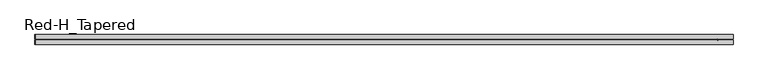
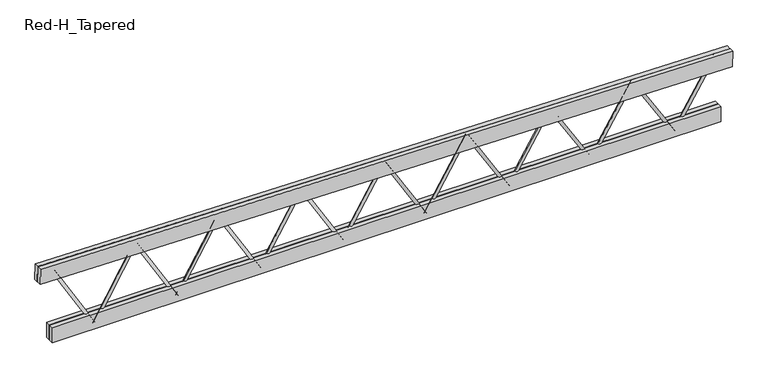
"""IFC4 building model written with IfcOpenShell, lengths in millimetres: beam geometry, Construction_Frames_RedBuilt_Openweb_Red-H_Tapered : Red-H_Tapered."""

from ifc_helpers import new_model, si_unit, point, frame, origin, origin_2d, place, context, project, spatial, polyline, circle_curve, trimmed, segment, composite_curve, outline, extrude, source, transform, mapped, element, save


def red_h_tapered_639e8230(model_context):
    return source(origin(), model_context, "Body", "SweptSolid", [
        extrude(outline(composite_curve([segment(trimmed(circle_curve(origin_2d(), 12.7), [point((0.0, 12.7))], [point((0.0, -12.7))], False, "CARTESIAN"), True, "CONTINUOUS"), segment(trimmed(circle_curve(origin_2d(), 12.7), [point((0.0, -12.7))], [point((0.0, 12.7))], False, "CARTESIAN"), True, "CONTINUOUS")], self_intersect=False)), frame((2514.6356775, 0.0, -367.0101562), z_axis=(0.5238075847033234, 0.0, 0.8518366123895301), x_axis=(0.0, -1.0, 0.0)), (0.0, 0.0, 1.0), 685.812269),
        extrude(outline(composite_curve([segment(trimmed(circle_curve(origin_2d(), 12.7), [point((0.0, -12.7))], [point((0.0, 12.6999999))], False, "CARTESIAN"), True, "CONTINUOUS"), segment(trimmed(circle_curve(origin_2d(), 12.7), [point((0.0, 12.6999999))], [point((0.0, -12.7))], False, "CARTESIAN"), True, "CONTINUOUS")], self_intersect=False)), frame((2514.6356775, 0.0, -367.0101562), z_axis=(-0.5212365661564216, 0.0, 0.8534122345627947), x_axis=(0.0, -1.0, 0.0)), (0.0, 0.0, 1.0), 689.1950633),
        extrude(outline(composite_curve([segment(trimmed(circle_curve(origin_2d(), 12.7), [point((0.0, 12.7))], [point((0.0, -12.6999999))], False, "CARTESIAN"), True, "CONTINUOUS"), segment(trimmed(circle_curve(origin_2d(), 12.7), [point((0.0, -12.6999999))], [point((0.0, 12.7))], False, "CARTESIAN"), True, "CONTINUOUS")], self_intersect=False)), frame((1796.168341, 0.0, -367.0101562), z_axis=(0.5212365661564208, 0.0, 0.8534122345627951), x_axis=(0.0, -1.0, 0.0)), (0.0, 0.0, 1.0), 689.1950633),
        extrude(outline(composite_curve([segment(trimmed(circle_curve(origin_2d(), 12.7), [point((0.0, -12.7))], [point((0.0, 12.7000001))], False, "CARTESIAN"), True, "CONTINUOUS"), segment(trimmed(circle_curve(origin_2d(), 12.7), [point((0.0, 12.7000001))], [point((0.0, -12.7))], False, "CARTESIAN"), True, "CONTINUOUS")], self_intersect=False)), frame((1796.168341, 0.0, -367.0101562), z_axis=(-0.5186860157662654, 0.0, 0.854964804567134), x_axis=(0.0, -1.0, 0.0)), (0.0, 0.0, 1.0), 692.584063),
        extrude(outline(composite_curve([segment(trimmed(circle_curve(origin_2d(), 12.7), [point((0.0, 12.7))], [point((0.0, -12.7))], False, "CARTESIAN"), True, "CONTINUOUS"), segment(trimmed(circle_curve(origin_2d(), 12.7), [point((0.0, -12.7))], [point((0.0, 12.7))], False, "CARTESIAN"), True, "CONTINUOUS")], self_intersect=False)), frame((1077.7010046, 0.0, -367.0101562), z_axis=(0.5186860157662644, 0.0, 0.8549648045671345), x_axis=(0.0, -1.0, 0.0)), (0.0, 0.0, 1.0), 692.584063),
        extrude(outline(composite_curve([segment(trimmed(circle_curve(origin_2d(), 12.7), [point((0.0, -12.7))], [point((0.0, 12.7))], False, "CARTESIAN"), True, "CONTINUOUS"), segment(trimmed(circle_curve(origin_2d(), 12.7), [point((0.0, 12.7))], [point((0.0, -12.7))], False, "CARTESIAN"), True, "CONTINUOUS")], self_intersect=False)), frame((1077.7010046, 0.0, -367.0101562), z_axis=(-0.5161557699811348, 0.0, 0.8564947291812028), x_axis=(0.0, -1.0, 0.0)), (0.0, 0.0, 1.0), 695.9791774),
        extrude(outline(composite_curve([segment(trimmed(circle_curve(origin_2d(), 12.7), [point((0.0, 12.7))], [point((0.0, -12.7))], False, "CARTESIAN"), True, "CONTINUOUS"), segment(trimmed(circle_curve(origin_2d(), 12.7), [point((0.0, -12.7))], [point((0.0, 12.7))], False, "CARTESIAN"), True, "CONTINUOUS")], self_intersect=False)), frame((359.2336682, 0.0, -367.0101562), z_axis=(0.5161557699811353, 0.0, 0.8564947291812025), x_axis=(0.0, -1.0, 0.0)), (0.0, 0.0, 1.0), 695.9791774),
        extrude(outline(composite_curve([segment(trimmed(circle_curve(origin_2d(), 12.7), [point((0.0, -12.7000001))], [point((0.0, 12.7))], False, "CARTESIAN"), True, "CONTINUOUS"), segment(trimmed(circle_curve(origin_2d(), 12.7), [point((0.0, 12.7))], [point((0.0, -12.7000001))], False, "CARTESIAN"), True, "CONTINUOUS")], self_intersect=False)), frame((359.2336682, 0.0, -367.0101562), z_axis=(-0.5136456648662082, 0.0, 0.8580024073183892), x_axis=(0.0, -1.0, 0.0)), (0.0, 0.0, 1.0), 699.3803176),
        extrude(outline(composite_curve([segment(trimmed(circle_curve(origin_2d(), 12.7), [point((0.0, -12.7))], [point((0.0, 12.7000001))], False, "CARTESIAN"), True, "CONTINUOUS"), segment(trimmed(circle_curve(origin_2d(), 12.7), [point((0.0, 12.7000001))], [point((0.0, -12.7))], False, "CARTESIAN"), True, "CONTINUOUS")], self_intersect=False)), frame((-359.2336682, 0.0, -367.0101562), z_axis=(0.5136456648661768, 0.0, 0.858002407318408), x_axis=(0.0, -1.0, 0.0)), (0.0, 0.0, 1.0), 699.3803176),
        extrude(outline(composite_curve([segment(trimmed(circle_curve(origin_2d(), 12.7), [point((0.0, 12.7))], [point((0.0, -12.7))], False, "CARTESIAN"), True, "CONTINUOUS"), segment(trimmed(circle_curve(origin_2d(), 12.7), [point((0.0, -12.7))], [point((0.0, 12.7))], False, "CARTESIAN"), True, "CONTINUOUS")], self_intersect=False)), frame((-359.2336682, 0.0, -367.0101562), z_axis=(-0.5111555362037679, 0.0, 0.8594882301743513), x_axis=(0.0, -1.0, 0.0)), (0.0, 0.0, 1.0), 702.7873959),
        extrude(outline(composite_curve([segment(trimmed(circle_curve(origin_2d(), 12.7), [point((0.0, -12.7000001))], [point((0.0, 12.7))], False, "CARTESIAN"), True, "CONTINUOUS"), segment(trimmed(circle_curve(origin_2d(), 12.7), [point((0.0, 12.7))], [point((0.0, -12.7000001))], False, "CARTESIAN"), True, "CONTINUOUS")], self_intersect=False)), frame((-1077.7010046, 0.0, -367.0101562), z_axis=(0.5111555362037662, 0.0, 0.8594882301743523), x_axis=(0.0, -1.0, 0.0)), (0.0, 0.0, 1.0), 702.7873959),
        extrude(outline(composite_curve([segment(trimmed(circle_curve(origin_2d(), 12.7), [point((0.0, 12.7))], [point((0.0, -12.7))], False, "CARTESIAN"), True, "CONTINUOUS"), segment(trimmed(circle_curve(origin_2d(), 12.7), [point((0.0, -12.7))], [point((0.0, 12.7))], False, "CARTESIAN"), True, "CONTINUOUS")], self_intersect=False)), frame((-1077.7010046, 0.0, -367.0101562), z_axis=(-0.5086852195886402, 0.0, 0.8609525813725497), x_axis=(0.0, -1.0, 0.0)), (0.0, 0.0, 1.0), 706.2003266),
        extrude(outline(composite_curve([segment(trimmed(circle_curve(origin_2d(), 12.7), [point((0.0, -12.7))], [point((0.0, 12.6999999))], False, "CARTESIAN"), True, "CONTINUOUS"), segment(trimmed(circle_curve(origin_2d(), 12.7), [point((0.0, 12.6999999))], [point((0.0, -12.7))], False, "CARTESIAN"), True, "CONTINUOUS")], self_intersect=False)), frame((-1796.168341, 0.0, -367.0101562), z_axis=(0.5086852195886533, 0.0, 0.860952581372542), x_axis=(0.0, -1.0, 0.0)), (0.0, 0.0, 1.0), 706.2003266),
        extrude(outline(composite_curve([segment(trimmed(circle_curve(origin_2d(), 12.7), [point((0.0, 12.6999999))], [point((0.0, -12.7000001))], False, "CARTESIAN"), True, "CONTINUOUS"), segment(trimmed(circle_curve(origin_2d(), 12.7), [point((0.0, -12.7000001))], [point((0.0, 12.6999999))], False, "CARTESIAN"), True, "CONTINUOUS")], self_intersect=False)), frame((-1796.168341, 0.0, -367.0101562), z_axis=(-0.5062345505185007, 0.0, 0.8623958371080716), x_axis=(0.0, -1.0, 0.0)), (0.0, 0.0, 1.0), 709.6190251),
        extrude(outline(composite_curve([segment(trimmed(circle_curve(origin_2d(), 12.7), [point((0.0, -12.6999999))], [point((0.0, 12.7000001))], False, "CARTESIAN"), True, "CONTINUOUS"), segment(trimmed(circle_curve(origin_2d(), 12.7), [point((0.0, 12.7000001))], [point((0.0, -12.6999999))], False, "CARTESIAN"), True, "CONTINUOUS")], self_intersect=False)), frame((-2514.6356775, 0.0, -367.0101562), z_axis=(0.506234550518489, 0.0, 0.8623958371080784), x_axis=(0.0, -1.0, 0.0)), (0.0, 0.0, 1.0), 709.6190251),
        extrude(outline(composite_curve([segment(trimmed(circle_curve(origin_2d(), 12.7), [point((0.0, 12.7))], [point((0.0, -12.7))], False, "CARTESIAN"), True, "CONTINUOUS"), segment(trimmed(circle_curve(origin_2d(), 12.7), [point((0.0, -12.7))], [point((0.0, 12.7))], False, "CARTESIAN"), True, "CONTINUOUS")], self_intersect=False)), frame((-2514.6356775, 0.0, -367.0101562), z_axis=(-0.5038033644797567, 0.0, 0.8638183662893939), x_axis=(0.0, -1.0, 0.0)), (0.0, 0.0, 1.0), 713.0434085),
        extrude(outline(polyline([(-2899.2693457, -41.275), (-2899.2693457, -3.175), (2899.2693457, -3.175), (2899.2693457, -41.275), (-2899.2693457, -41.275)])), frame((0.0, 0.0, -386.0601562), z_axis=(0.0, 0.0, 1.0), x_axis=(1.0, 0.0, 0.0)), (0.0, 0.0, 1.0), 139.7),
        extrude(outline(polyline([(-2899.2693457, 3.175), (-2899.2693457, 41.275), (2899.2693457, 41.275), (2899.2693457, 3.175), (-2899.2693457, 3.175)])), frame((0.0, 0.0, -386.0601562), z_axis=(0.0, 0.0, 1.0), x_axis=(1.0, 0.0, 0.0)), (0.0, 0.0, 1.0), 139.7),
        extrude(outline(polyline([(0.0, -38.1), (0.0, 0.0), (6002.5985939, 0.0), (6002.5985939, -38.1), (0.0, -38.1)])), frame((-3003.2339083, -3.175, 185.4598565), z_axis=(0.016926002698829056, 0.0, 0.9998567449553157), x_axis=(0.9998567449553157, 0.0, -0.016926002698829056)), (0.0, 0.0, 1.0), 139.7),
        extrude(outline(polyline([(0.0, -38.1), (0.0, 0.0), (6002.5985939, 0.0), (6002.5985939, -38.1), (0.0, -38.1)])), frame((-3003.2339083, 41.275, 185.4598565), z_axis=(0.016926002698829056, 0.0, 0.9998567449553157), x_axis=(0.9998567449553157, 0.0, -0.016926002698829056)), (0.0, 0.0, 1.0), 139.7),
    ])


if __name__ == "__main__":
    model = new_model("IFC4")
    model_context = context("Model", 3, world=origin())
    ifc_project = project(units=[si_unit("LENGTHUNIT", "METRE", prefix="MILLI")], contexts=[model_context])
    site = spatial("IfcSite", under=ifc_project)
    building = spatial("IfcBuilding", under=site)
    placement = place(None, origin())
    red_h_tapered_shape = red_h_tapered_639e8230(model_context)
    element("IfcBeam", 1, ObjectType="Construction_Frames_RedBuilt_Openweb_Red-H_Tapered : Red-H_Tapered", at=placement, inside=building, context=model_context, shape_type="MappedRepresentation", body=[
        mapped(red_h_tapered_shape, transform((0.0, 0.0, 0.0), x_axis=(1.0, 0.0, 0.0), y_axis=(0.0, 1.0, 0.0), z_axis=(0.0, 0.0, 1.0))),
    ])
    save(model, "model.ifc")

# Revit data of these elements
# Type "Construction_Frames_RedBuilt_Openweb_Red-H_Tapered : Red-H_Tapered"
#   Youtube clip = ""
#   Weight Net (Kg) = "0"
#   Webs = "Up to 2\" diameter tubular steel"
#   Uniformat II Description = ""
#   Uniformat II Code = ""
#   Uniclass 2015 Name = "Softwood trusses"
#   Uniclass 2015 Code = "Pr_20_85_90_81"
#   Uniclass 2.0 Description = "Structural Framing Systems"
#   Uniclass 2.0 Code = "SS-15-10-75"
#   Uniclass 1.4 Description = "Trusses"
#   Uniclass 1.4 Code = "L3523"
#   UNSPSC Code = "30103606"
#   Technical description = "http://www.redbuilt.com/reference/literature-and-other-resources"
#   Region South America = "None"
#   Region Oceania = "None"
#   Region North America = "US"
#   Region Middle East = "None"
#   Region Europe = "None"
#   Region Asia = "None"
#   Region Antarctica = "None"
#   Region Africa = "None"
#   QR code = "http://bimobject.com/redbuilt/product/redbuilt-0003"
#   Product url = "http://www.redbuilt.com/products/default.aspx?id=2"
#   Product group = "Wood Trusses"
#   Product family = "Construction"
#   Product data url = "https://bimobject.com/redbuilt/product/redbuilt-0003"
#   Product certification = ""
#   Product SKU = "redbuilt-0003"
#   Product Page URL = "http://www.redbuilt.com/commercial-systems/red-m-red-h-open-web-trusses"
#   Product Guid = "2c5793f2-6ffb-4665-b825-cf90c048e711"
#   Product Documentation Link = "http://www.redbuilt.com/documents/OW_Guide_2017_07_LowRes_wLinks.pdf"
#   OmniClass Description = "Wood Trusses"
#   OmniClass Code = "23-13 35 19 13 17"
#   NBS Reference Description = ""
#   NBS Reference Code = ""
#   Material secondary = "Steel"
#   Material main = "CHARRED WOOD"
#   Masterformat 2014 Description = "Metal-Web Wood Joists"
#   Masterformat 2014 Code = "06 17 36"
#   Manufacturer name = "RedBuilt"
#   Manufacturer country = "United States"
#   Installation instructions = "http://www.redbuilt.com/documents/Installation_Sheets_Open-Web.pdf"
#   IFC Classification = ""
#   EAN code = ""
#   Design country = "United States"
#   Product Information = "http://redbuilt.com/products/default.aspx?id=2"
#   Model = "Red-H-Tapered"
#   Manufacturer URL = "http://redbuilt.com/"
#   Manufacturer = "RedBuilt™"
#   Description = "Open Web Truss"
#   Date of publishing = "8/17/2010"
#   Contact us = "http://redbuilt.com/contact/"
#   Chords = "Double 1½\" x 5½\" MSR lumber"
#   COBIe Type Category = ""
#   Brand url = "http://www.redbuilt.com"
#   BIMobject main category code = "construction"
#   BIMobject main category = "Construction"
#   BIMobject category code = "construction-frames-trusses"
#   BIMobject category = "Frames & Trusses"
#   Web Radius = 0' - 0 1/2"
#   Web Layout Offset Start [instance default] = 0' - 5"
#   Web Layout Offset End [instance default] = 0' - 5"
#   Web Diameter = 0' - 1"
#   TotalLength [instance default] = 20' - 0"
#   Span Minimum = 4' - 0"
#   Span Maximum = 70' - 0"
#   Span Limit [instance default] = 20' - 0"
#   Nominal width = 0' - 0"
#   Nominal height = 0' - 0"
#   Inner Depth Top [instance default] = 0' - 2.76372"
#   Depth Start [instance default] = 6' - 0"
#   Top Chord Length [instance default] = 20' - 1.19701"
#   TC Extension Start Aux [instance default] = 0' - 0"
#   TC Extension End Aux [instance default] = 0' - 0"
#   T-B Chord Length Difference L [instance default] = 0' - 4"
#   T-B Chord Length Difference [instance default] = 0' - 4"
#   Height 2 [instance default] = 6' - 0"
#   Depth Minimum at Wall = 2' - 0"
#   Depth Maximum at Wall = 6' - 0"
#   Depth Lower End [instance default] = 2' - 0"
#   Depth Higher End [instance default] = 6' - 0"
#   Depth End [instance default] = 2' - 0"
#   Depth 2 [instance default] = 2' - 0"
#   Chord Width = 0' - 3 1/4"
#   Chord Thickness = 0' - 1 1/2"
#   Chord Depth = 0' - 5 1/2"
#   Offset Start [instance default] = 0' - 0"
#   TC Extension Start [instance default] = 0' - 0"
#   End Panel = 0' - 5"
#   Offset End [instance default] = 0' - 0"
#   TC Extension End [instance default] = 0' - 0"
#   Length [instance default] = 20' - 0"
#   Angle [instance default] = 5.71059°
#   Span Limit Warning [instance default] = no
#   Edition number = 1
#   Top Bearing Start [instance default] = yes
#   Top Bearing End [instance default] = yes
#   Bottom Bearing Start [instance default] = no
#   Bottom Bearing End [instance default] = no
#   8 Panels [instance default] = yes
#   16 Panels [instance default] = no
#   12 Panels [instance default] = no
#   Web Material = RedBuilt-Steel, Galvanized
#   Clip Material = RedBuilt-Steel, Galvanized
#   Chords Material = WOOD-OAKFIRE
#   URL = ""
#   Assembly Code = ""
# Element 1 (IfcBeam, "Construction_Frames_RedBuilt_Openweb_Red-H_Tapered : Red-H_Tapered")
#   TotalLength = 19' - 8.28892"
#   Span Limit = 19' - 8.28892"
#   Inner Depth Top = 0' - 2.75039"
#   Depth Start = 5' - 0"
#   Top Chord Length = 19' - 8.32278"
#   Height 2 = 5' - 0"
#   Depth Higher End = 5' - 0"
#   Depth 2 = 0' - 4"
#   Angle = 0.969835°
#   Materials on its faces: "RedBuilt-Steel, Galvanized", "WOOD-OAKFIRE"
# Materials
#   "RedBuilt-Steel, Galvanized": class "Metal", colour RGB 164 172 176, transparency 0, Manufacturer = "RedBuilt. LLC", Comments = "Openweb Metal Web", URL = "http://www.redbuilt.com/", Description = "Galvanized steel", Cost = 0
#   "WOOD-OAKFIRE": class "Wood", colour RGB 198 202 183, transparency 0, Description = "Generic wood", Cost = 0
